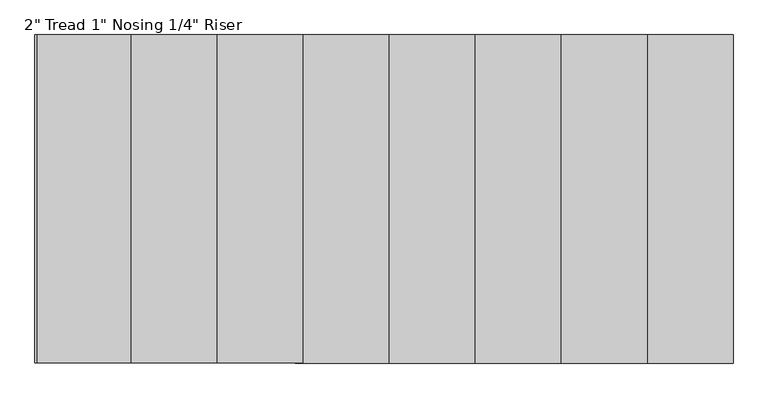
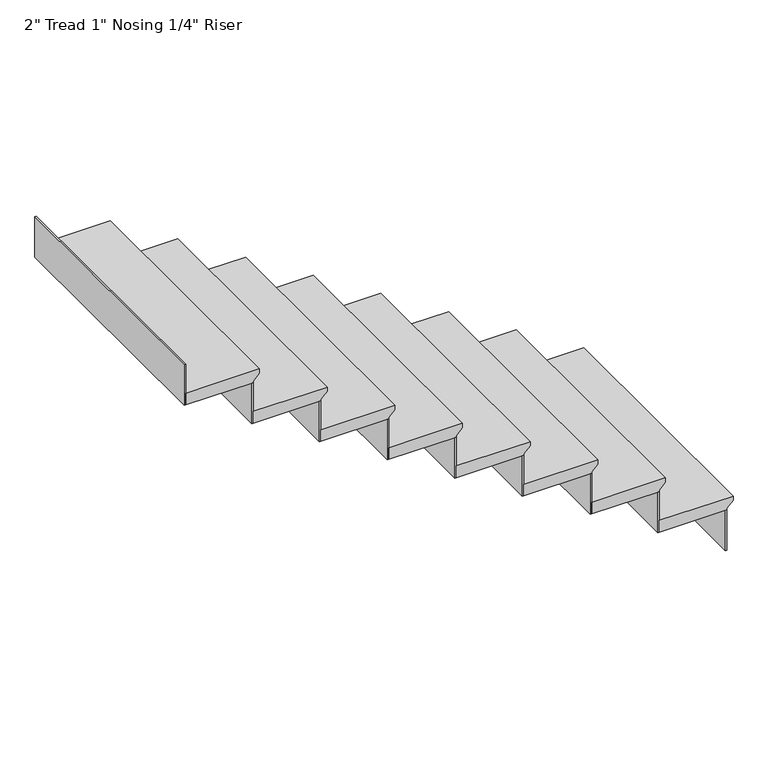
"""IFC4 building model written with IfcOpenShell, lengths in millimetres: stair flight geometry."""

from ifc_helpers import new_model, si_unit, origin, place, context, project, spatial, faceted_brep, source, transform, mapped, element, save


def stair_flight_e4acb099(model_context):
    return source(origin(), model_context, "Body", "Brep", [
        faceted_brep([(665956.388677, -549416.0413841, 1752.0851351), (665956.388677, -549416.0413841, 1771.1351351), (665956.388677, -550482.8413841, 1771.1351351), (665956.388677, -550482.8413841, 1752.0851351), (665930.988677, -549416.0413841, 1726.6851351), (665930.988677, -550482.8413841, 1726.6851351), (665651.588677, -549416.0413841, 1771.1351351), (665651.588677, -550482.8413841, 1771.1351351), (665930.988677, -550482.8413841, 1720.3351351), (665651.588677, -550482.8413841, 1720.3351351), (665651.588677, -549416.0413841, 1720.3351351), (665930.988677, -549416.0413841, 1720.3351351)], [[[0, 1, 2, 3]], [[4, 0, 3, 5]], [[2, 1, 6, 7]], [[8, 9, 10, 11]], [[2, 7, 9, 8, 5, 3]], [[8, 11, 4, 5]], [[6, 1, 0, 4, 11, 10]], [[7, 6, 10, 9]]]),
        faceted_brep([(665930.988677, -549416.0413841, 1720.3351351), (665930.988677, -549416.0413841, 1543.2216216), (665924.638677, -549416.0413841, 1543.2216216), (665924.638677, -549416.0413841, 1720.3351351), (665930.988677, -550482.8413841, 1720.3351351), (665924.638677, -550482.8413841, 1720.3351351), (665924.638677, -550482.8413841, 1543.2216216), (665930.988677, -550482.8413841, 1543.2216216)], [[[0, 1, 2, 3]], [[4, 5, 6, 7]], [[1, 0, 4, 7]], [[2, 1, 7, 6]], [[3, 2, 6, 5]], [[0, 3, 5, 4]]]),
        faceted_brep([(665651.588677, -549416.0413841, 1897.4486486), (665651.588677, -549416.0413841, 1720.3351351), (665645.238677, -549416.0413841, 1720.3351351), (665645.238677, -549416.0413841, 1897.4486486), (665651.588677, -550482.8413841, 1897.4486486), (665645.238677, -550482.8413841, 1897.4486486), (665645.238677, -550482.8413841, 1720.3351351), (665651.588677, -550482.8413841, 1720.3351351)], [[[0, 1, 2, 3]], [[4, 5, 6, 7]], [[1, 0, 4, 7]], [[2, 1, 7, 6]], [[3, 2, 6, 5]], [[0, 3, 5, 4]]]),
        faceted_brep([(665676.988677, -550482.8413841, 1948.2486486), (665676.988677, -549416.0413841, 1948.2486486), (665372.188677, -549416.0413841, 1948.2486486), (665372.188677, -550482.8413841, 1948.2486486), (665651.588677, -550482.8413841, 1897.4486486), (665372.188677, -550482.8413841, 1897.4486486), (665372.188677, -549416.0413841, 1897.4486486), (665651.588677, -549416.0413841, 1897.4486486), (665651.588677, -550482.8413841, 1903.7986486), (665676.988677, -550482.8413841, 1929.1986486), (665651.588677, -549416.0413841, 1903.7986486), (665676.988677, -549416.0413841, 1929.1986486)], [[[0, 1, 2, 3]], [[4, 5, 6, 7]], [[0, 3, 5, 4, 8, 9]], [[4, 7, 10, 8]], [[2, 1, 11, 10, 7, 6]], [[3, 2, 6, 5]], [[11, 1, 0, 9]], [[10, 11, 9, 8]]]),
        faceted_brep([(665372.188677, -549416.0413841, 2074.5621622), (665372.188677, -549416.0413841, 1897.4486486), (665365.838677, -549416.0413841, 1897.4486486), (665365.838677, -549416.0413841, 2074.5621622), (665372.188677, -550482.8413841, 2074.5621622), (665365.838677, -550482.8413841, 2074.5621622), (665365.838677, -550482.8413841, 1897.4486486), (665372.188677, -550482.8413841, 1897.4486486)], [[[0, 1, 2, 3]], [[4, 5, 6, 7]], [[1, 0, 4, 7]], [[2, 1, 7, 6]], [[3, 2, 6, 5]], [[0, 3, 5, 4]]]),
        faceted_brep([(665397.588677, -550482.8413841, 2125.3621622), (665397.588677, -549416.0413841, 2125.3621622), (665092.788677, -549416.0413841, 2125.3621622), (665092.788677, -550482.8413841, 2125.3621622), (665372.188677, -550482.8413841, 2074.5621622), (665092.788677, -550482.8413841, 2074.5621622), (665092.788677, -549416.0413841, 2074.5621622), (665372.188677, -549416.0413841, 2074.5621622), (665372.188677, -550482.8413841, 2080.9121622), (665397.588677, -550482.8413841, 2106.3121622), (665372.188677, -549416.0413841, 2080.9121622), (665397.588677, -549416.0413841, 2106.3121622)], [[[0, 1, 2, 3]], [[4, 5, 6, 7]], [[0, 3, 5, 4, 8, 9]], [[4, 7, 10, 8]], [[2, 1, 11, 10, 7, 6]], [[3, 2, 6, 5]], [[11, 1, 0, 9]], [[10, 11, 9, 8]]]),
        faceted_brep([(665092.788677, -549416.0413841, 2251.6756757), (665092.788677, -549416.0413841, 2074.5621622), (665086.438677, -549416.0413841, 2074.5621622), (665086.438677, -549416.0413841, 2251.6756757), (665092.788677, -550482.8413841, 2251.6756757), (665086.438677, -550482.8413841, 2251.6756757), (665086.438677, -550482.8413841, 2074.5621622), (665092.788677, -550482.8413841, 2074.5621622)], [[[0, 1, 2, 3]], [[4, 5, 6, 7]], [[1, 0, 4, 7]], [[2, 1, 7, 6]], [[3, 2, 6, 5]], [[0, 3, 5, 4]]]),
        faceted_brep([(665118.188677, -550482.8413841, 2302.4756757), (665118.188677, -549416.0413841, 2302.4756757), (664813.388677, -549416.0413841, 2302.4756757), (664813.388677, -550482.8413841, 2302.4756757), (665092.788677, -550482.8413841, 2251.6756757), (664813.388677, -550482.8413841, 2251.6756757), (664813.388677, -549416.0413841, 2251.6756757), (665092.788677, -549416.0413841, 2251.6756757), (665092.788677, -550482.8413841, 2258.0256757), (665118.188677, -550482.8413841, 2283.4256757), (665092.788677, -549416.0413841, 2258.0256757), (665118.188677, -549416.0413841, 2283.4256757)], [[[0, 1, 2, 3]], [[4, 5, 6, 7]], [[0, 3, 5, 4, 8, 9]], [[4, 7, 10, 8]], [[2, 1, 11, 10, 7, 6]], [[3, 2, 6, 5]], [[11, 1, 0, 9]], [[10, 11, 9, 8]]]),
        faceted_brep([(664813.388677, -549416.0413841, 2428.7891892), (664813.388677, -549416.0413841, 2251.6756757), (664807.038677, -549416.0413841, 2251.6756757), (664807.038677, -549416.0413841, 2428.7891892), (664813.388677, -550482.8413841, 2428.7891892), (664807.038677, -550482.8413841, 2428.7891892), (664807.038677, -550482.8413841, 2251.6756757), (664813.388677, -550482.8413841, 2251.6756757)], [[[0, 1, 2, 3]], [[4, 5, 6, 7]], [[1, 0, 4, 7]], [[2, 1, 7, 6]], [[3, 2, 6, 5]], [[0, 3, 5, 4]]]),
        faceted_brep([(664838.788677, -550482.8413841, 2479.5891892), (664838.788677, -549416.0413841, 2479.5891892), (664533.988677, -549416.0413841, 2479.5891892), (664533.988677, -550482.8413841, 2479.5891892), (664813.388677, -550482.8413841, 2428.7891892), (664533.988677, -550482.8413841, 2428.7891892), (664533.988677, -549416.0413841, 2428.7891892), (664813.388677, -549416.0413841, 2428.7891892), (664813.388677, -550482.8413841, 2435.1391892), (664838.788677, -550482.8413841, 2460.5391892), (664813.388677, -549416.0413841, 2435.1391892), (664838.788677, -549416.0413841, 2460.5391892)], [[[0, 1, 2, 3]], [[4, 5, 6, 7]], [[0, 3, 5, 4, 8, 9]], [[4, 7, 10, 8]], [[2, 1, 11, 10, 7, 6]], [[3, 2, 6, 5]], [[11, 1, 0, 9]], [[10, 11, 9, 8]]]),
        faceted_brep([(664533.988677, -549416.0413841, 2605.9027027), (664533.988677, -549416.0413841, 2428.7891892), (664527.638677, -549416.0413841, 2428.7891892), (664527.638677, -549416.0413841, 2605.9027027), (664533.988677, -550482.8413841, 2605.9027027), (664527.638677, -550482.8413841, 2605.9027027), (664527.638677, -550482.8413841, 2428.7891892), (664533.988677, -550482.8413841, 2428.7891892)], [[[0, 1, 2, 3]], [[4, 5, 6, 7]], [[1, 0, 4, 7]], [[2, 1, 7, 6]], [[3, 2, 6, 5]], [[0, 3, 5, 4]]]),
        faceted_brep([(664559.388677, -550482.8413841, 2656.7027027), (664559.388677, -549416.0413841, 2656.7027027), (664254.588677, -549416.0413841, 2656.7027027), (664254.588677, -550482.8413841, 2656.7027027), (664533.988677, -550482.8413841, 2605.9027027), (664254.588677, -550482.8413841, 2605.9027027), (664254.588677, -549416.0413841, 2605.9027027), (664533.988677, -549416.0413841, 2605.9027027), (664533.988677, -550482.8413841, 2612.2527027), (664559.388677, -550482.8413841, 2637.6527027), (664533.988677, -549416.0413841, 2612.2527027), (664559.388677, -549416.0413841, 2637.6527027)], [[[0, 1, 2, 3]], [[4, 5, 6, 7]], [[0, 3, 5, 4, 8, 9]], [[4, 7, 10, 8]], [[2, 1, 11, 10, 7, 6]], [[3, 2, 6, 5]], [[11, 1, 0, 9]], [[10, 11, 9, 8]]]),
        faceted_brep([(664254.588677, -549416.0413841, 2783.0162162), (664254.588677, -549416.0413841, 2605.9027027), (664248.238677, -549416.0413841, 2605.9027027), (664248.238677, -549416.0413841, 2783.0162162), (664254.588677, -550482.8413841, 2783.0162162), (664248.238677, -550482.8413841, 2783.0162162), (664248.238677, -550482.8413841, 2605.9027027), (664254.588677, -550482.8413841, 2605.9027027)], [[[0, 1, 2, 3]], [[4, 5, 6, 7]], [[1, 0, 4, 7]], [[2, 1, 7, 6]], [[3, 2, 6, 5]], [[0, 3, 5, 4]]]),
        faceted_brep([(664279.988677, -550482.8413841, 2833.8162162), (664279.988677, -549416.0413841, 2833.8162162), (663975.188677, -549416.0413841, 2833.8162162), (663975.188677, -550482.8413841, 2833.8162162), (664254.588677, -550482.8413841, 2783.0162162), (663975.188677, -550482.8413841, 2783.0162162), (663975.188677, -549416.0413841, 2783.0162162), (664254.588677, -549416.0413841, 2783.0162162), (664254.588677, -550482.8413841, 2789.3662162), (664279.988677, -550482.8413841, 2814.7662162), (664254.588677, -549416.0413841, 2789.3662162), (664279.988677, -549416.0413841, 2814.7662162)], [[[0, 1, 2, 3]], [[4, 5, 6, 7]], [[0, 3, 5, 4, 8, 9]], [[4, 7, 10, 8]], [[2, 1, 11, 10, 7, 6]], [[3, 2, 6, 5]], [[11, 1, 0, 9]], [[10, 11, 9, 8]]]),
        faceted_brep([(663695.788677, -549416.0413841, 3137.2432432), (663695.788677, -549416.0413841, 2960.1297297), (663689.438677, -549416.0413841, 2960.1297297), (663689.438677, -549416.0413841, 3137.2432432), (663695.788677, -550482.8413841, 3137.2432432), (663689.438677, -550482.8413841, 3137.2432432), (663689.438677, -550482.8413841, 2960.1297297), (663695.788677, -550482.8413841, 2960.1297297)], [[[0, 1, 2, 3]], [[4, 5, 6, 7]], [[1, 0, 4, 7]], [[2, 1, 7, 6]], [[3, 2, 6, 5]], [[0, 3, 5, 4]]]),
        faceted_brep([(663975.188677, -549416.0413841, 2960.1297297), (663975.188677, -549416.0413841, 2783.0162162), (663968.838677, -549416.0413841, 2783.0162162), (663968.838677, -549416.0413841, 2960.1297297), (663975.188677, -550482.8413841, 2960.1297297), (663968.838677, -550482.8413841, 2960.1297297), (663968.838677, -550482.8413841, 2783.0162162), (663975.188677, -550482.8413841, 2783.0162162)], [[[0, 1, 2, 3]], [[4, 5, 6, 7]], [[1, 0, 4, 7]], [[2, 1, 7, 6]], [[3, 2, 6, 5]], [[0, 3, 5, 4]]]),
        faceted_brep([(664000.588677, -550482.8413841, 3010.9297297), (664000.588677, -549416.0413841, 3010.9297297), (663721.188677, -549416.0413841, 3010.9297297), (663695.788677, -549416.0413841, 3010.9297297), (663695.788677, -550482.8413841, 3010.9297297), (663975.188677, -550482.8413841, 2960.1297297), (663695.788677, -550482.8413841, 2960.1297297), (663695.788677, -549416.0413841, 2960.1297297), (663721.188677, -549416.0413841, 2960.1297297), (663975.188677, -549416.0413841, 2960.1297297), (663975.188677, -550482.8413841, 2966.4797297), (664000.588677, -550482.8413841, 2991.8797297), (663975.188677, -549416.0413841, 2966.4797297), (664000.588677, -549416.0413841, 2991.8797297)], [[[0, 1, 2, 3, 4]], [[5, 6, 7, 8, 9]], [[0, 4, 6, 5, 10, 11]], [[5, 9, 12, 10]], [[2, 1, 13, 12, 9, 8]], [[3, 2, 8, 7]], [[4, 3, 7, 6]], [[13, 1, 0, 11]], [[12, 13, 11, 10]]]),
    ])


if __name__ == "__main__":
    model = new_model("IFC4")
    model_context = context("Model", 3, world=origin())
    ifc_project = project(units=[si_unit("LENGTHUNIT", "METRE", prefix="MILLI")], contexts=[model_context])
    site = spatial("IfcSite", under=ifc_project)
    building = spatial("IfcBuilding", under=site)
    placement = place(None, origin())
    stair_flight_shape = stair_flight_e4acb099(model_context)
    element("IfcStairFlight", 1, ObjectType="2\" Tread 1\" Nosing 1/4\" Riser", at=placement, inside=building, context=model_context, shape_type="MappedRepresentation", body=[
        mapped(stair_flight_shape, transform((0.0, 0.0, 0.0), x_axis=(1.0, 0.0, 0.0), y_axis=(0.0, 1.0, 0.0), z_axis=(0.0, 0.0, 1.0))),
    ])
    save(model, "model.ifc")
